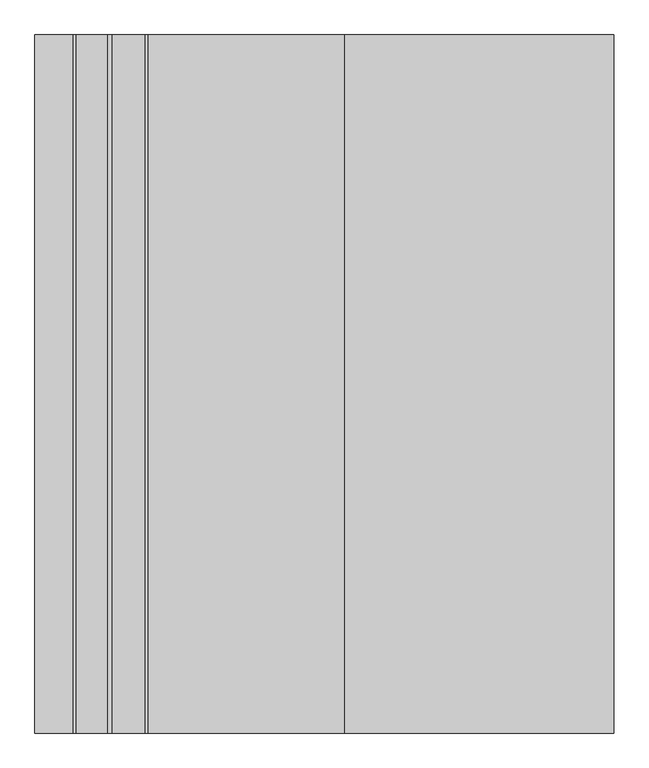
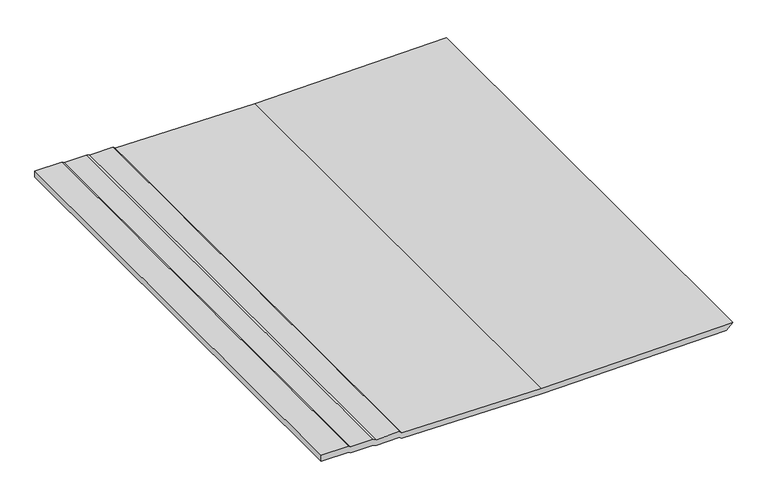
"""IFC4 building model written with IfcOpenShell, lengths in millimetres: proxy geometry, GRAVEL BALLAST002 15468 : GRAVEL BALLAST002 15468."""

from ifc_helpers import new_model, si_unit, frame, origin, place, context, project, spatial, polyline, outline, extrude, source, transform, mapped, element, save


def generic_models_deb63274(model_context):
    return source(origin(), model_context, "Body", "SweptSolid", [
        extrude(outline(polyline([(40274.2359465, -2672.3662777), (40269.9546965, -2663.6558285), (40269.9546965, -2573.0689144), (40264.2272345, -2560.2242751), (40265.8726652, -2466.2725277), (40258.462509, -2457.9990902), (40250.243759, -1894.9286556), (40261.546875, -1149.4367676), (40286.2851563, -1123.4630127), (40274.9820403, -1894.9286556), (40283.2007903, -2457.9990902), (40290.6109465, -2466.2725277), (40288.9655158, -2560.2242751), (40294.6929778, -2573.0689144), (40294.6929778, -2663.6558285), (40298.9742278, -2672.3662777), (40298.9742278, -2781.8657894), (40274.2359465, -2781.8657894), (40274.2359465, -2672.3662777)])), frame((0.0, -1052.6406573, 0.0), z_axis=(0.0, 1.0, 0.0), x_axis=(0.0, 0.0, 1.0)), (0.0, 0.0, 1.0), 2000.0),
    ])


if __name__ == "__main__":
    model = new_model("IFC4")
    model_context = context("Model", 3, world=origin())
    ifc_project = project(units=[si_unit("LENGTHUNIT", "METRE", prefix="MILLI")], contexts=[model_context])
    site = spatial("IfcSite", under=ifc_project)
    building = spatial("IfcBuilding", under=site)
    placement = place(None, origin())
    generic_models_shape = generic_models_deb63274(model_context)
    element("IfcBuildingElementProxy", 1, Name="GRAVEL BALLAST002 15468 : GRAVEL BALLAST002 15468", ObjectType="GRAVEL BALLAST002 15468 : GRAVEL BALLAST002 15468", at=placement, inside=building, context=model_context, shape_type="MappedRepresentation", body=[
        mapped(generic_models_shape, transform((0.0, 0.0, 0.0), x_axis=(1.0, 0.0, 0.0), y_axis=(0.0, 1.0, 0.0), z_axis=(0.0, 0.0, 1.0))),
    ])
    save(model, "model.ifc")

# Revit data of these elements
# Type "GRAVEL BALLAST002 15468 : GRAVEL BALLAST002 15468"
#   NameOverride = "GRAVEL BALLAST002"
# Element 1 (IfcBuildingElementProxy, "GRAVEL BALLAST002 15468 : GRAVEL BALLAST002 15468")
#   Materials on its faces: "GRAVEL BALLAST"
# Materials
#   "GRAVEL BALLAST": class "Unassigned", colour RGB 128 128 128, transparency 0, Cost = 0
